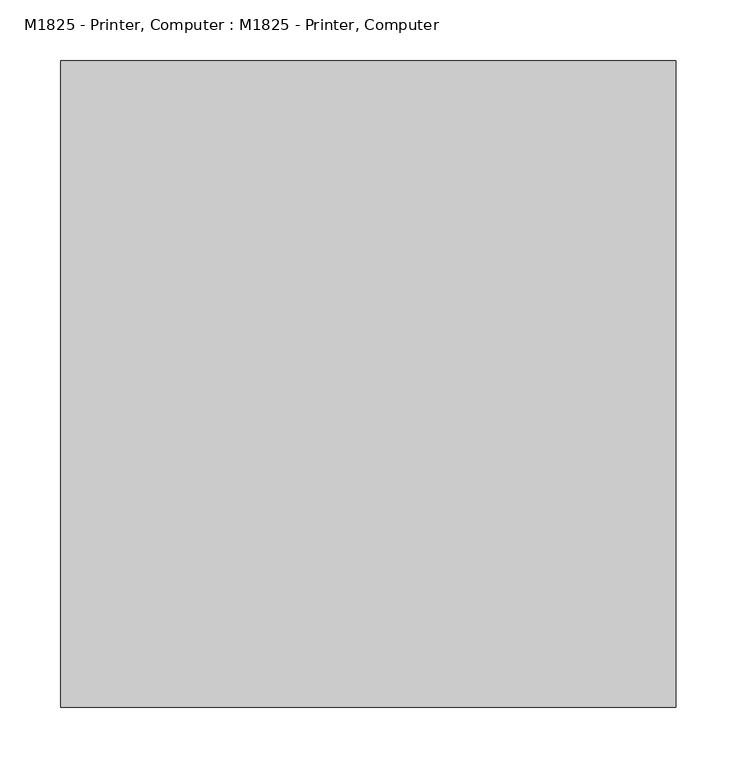
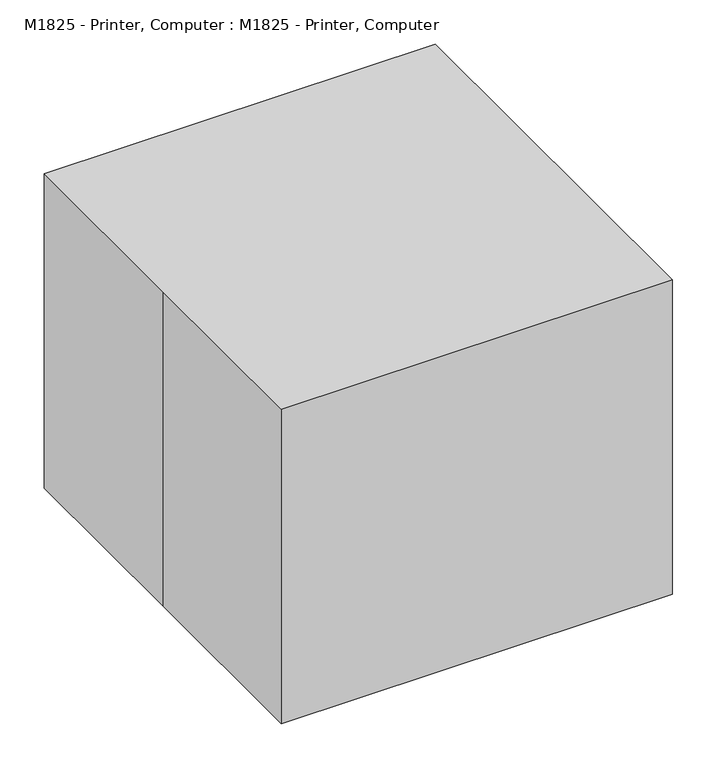
"""IFC4 building model written with IfcOpenShell, lengths in millimetres: proxy geometry, M1825 - Printer, Computer : M1825 - Printer, Computer."""

import ifcopenshell
import ifcopenshell.guid

model = None  # the IFC model being written
_history = None  # IfcOwnerHistory: only IFC2X3 demands one
_inside = {}  # id of a spatial element -> (the spatial element, [elements in it])
_under = {}  # id of a project, library or spatial element -> (it, [spatial elements below it])
_declared = {}  # id of a project -> (the project, [libraries it declares])
_typed = {}  # id of a type object -> (the type object, [elements of that type])
_made_of = {}  # id of a material, layer set ... -> (it, [elements and type objects made of it])


def new_model(schema):
    """Start an empty IFC model of exactly this schema.

    Asked for "IFC4X3", IfcOpenShell would pick the latest addendum, in which some entities
    have other attributes; the version numbers below select the first issue.
    IFC2X3 requires an IfcOwnerHistory on every rooted entity: one is made here for all.
    """
    global model, _history
    if schema == "IFC4X3":
        model = ifcopenshell.file(schema_version=(4, 3, 0, 0))
    else:
        model = ifcopenshell.file(schema=schema)
    _inside.clear()
    _under.clear()
    _declared.clear()
    _typed.clear()
    _made_of.clear()
    _history = None
    if model.schema == "IFC2X3":
        org = make("IfcOrganization", Name="unknown")
        user = make(
            "IfcPersonAndOrganization",
            ThePerson=make("IfcPerson", FamilyName="unknown"),
            TheOrganization=org,
        )
        app = make(
            "IfcApplication",
            ApplicationDeveloper=org,
            Version="unknown",
            ApplicationFullName="unknown",
            ApplicationIdentifier="unknown",
        )
        _history = make(
            "IfcOwnerHistory",
            OwningUser=user,
            OwningApplication=app,
            ChangeAction="ADDED",
            CreationDate=0,
        )
    return model


def make(cls, **values):
    """One entity of the class cls with the attributes given. An attribute that is None is left unset."""
    return model.create_entity(
        cls, **{name: value for name, value in values.items() if value is not None}
    )


def rooted(cls, **values):
    """An entity with a GlobalId (a new one), such as an element, a storey or a relation."""
    return make(cls, GlobalId=ifcopenshell.guid.new(), OwnerHistory=_history, **values)


def si_unit(unit_type, name, prefix=None):
    """IfcSIUnit, for example si_unit("LENGTHUNIT", "METRE", prefix="MILLI")."""
    return make("IfcSIUnit", UnitType=unit_type, Prefix=prefix, Name=name)


def assignment(units):
    """IfcUnitAssignment: the units of a project."""
    return None if units is None else make("IfcUnitAssignment", Units=units)


def point(xyz):
    """IfcCartesianPoint."""
    return None if xyz is None else make("IfcCartesianPoint", Coordinates=xyz)


def direction(xyz):
    """IfcDirection."""
    return None if xyz is None else make("IfcDirection", DirectionRatios=xyz)


def frame(location, z_axis=None, x_axis=None):
    """IfcAxis2Placement3D, a coordinate frame: its origin and axes. An axis left out is left unset."""
    return make(
        "IfcAxis2Placement3D",
        Location=point(location),
        Axis=direction(z_axis),
        RefDirection=direction(x_axis),
    )


def origin():
    """The frame at (0, 0, 0) with its axes left unset."""
    return frame((0.0, 0.0, 0.0))


def origin_with_axes():
    """The frame at (0, 0, 0) with the z axis (0, 0, 1) and the x axis (1, 0, 0) written out."""
    return frame((0.0, 0.0, 0.0), z_axis=(0.0, 0.0, 1.0), x_axis=(1.0, 0.0, 0.0))


def place(relative_to, where):
    """IfcLocalPlacement: puts the frame where relative to a parent placement (None: the world)."""
    return make(
        "IfcLocalPlacement", PlacementRelTo=relative_to, RelativePlacement=where
    )


def context(
    kind, dimensions, precision=None, world=None, true_north=None, identifier=None
):
    """IfcGeometricRepresentationContext, for example the 3D "Model" context."""
    return make(
        "IfcGeometricRepresentationContext",
        ContextIdentifier=identifier,
        ContextType=kind,
        CoordinateSpaceDimension=dimensions,
        Precision=precision,
        WorldCoordinateSystem=world,
        TrueNorth=true_north,
    )


def project(units=None, contexts=None):
    """IfcProject with its units and contexts."""
    return rooted(
        "IfcProject",
        Name="project",
        RepresentationContexts=contexts,
        UnitsInContext=assignment(units),
    )


def spatial(cls, under=None, at=None, **own):
    """A site, building, storey or space (cls), placed at a placement, below another one or the project."""
    s = rooted(cls, ObjectPlacement=at, **own)
    if under is not None:
        _under.setdefault(under.id(), (under, []))[1].append(s)
    return s


def polyline(points):
    """IfcPolyline through the points."""
    return make("IfcPolyline", Points=[point(p) for p in points])


def outline(outer, holes=None, kind="AREA"):
    """IfcArbitraryClosedProfileDef: a profile drawn as a closed curve; with holes, ...WithVoids."""
    if holes is None:
        return make("IfcArbitraryClosedProfileDef", ProfileType=kind, OuterCurve=outer)
    return make(
        "IfcArbitraryProfileDefWithVoids",
        ProfileType=kind,
        OuterCurve=outer,
        InnerCurves=holes,
    )


def extrude(swept, where, along, depth):
    """IfcExtrudedAreaSolid: the profile swept, set in the frame where, extruded along a direction by depth."""
    return make(
        "IfcExtrudedAreaSolid",
        SweptArea=swept,
        Position=where,
        ExtrudedDirection=direction(along),
        Depth=depth,
    )


def faces_of(points, faces, orient=None, outer=None):
    """IfcFace entities. A face is a list of loops; a loop is a list of indices into points, from 0.

    orient and outer hold one flag for each loop. By default every Orientation is true, the
    first loop of a face is its IfcFaceOuterBound and the others are IfcFaceBound.
    """
    made = []
    for i, loops in enumerate(faces):
        bounds = []
        for j, loop in enumerate(loops):
            is_outer = j == 0 if outer is None else outer[i][j]
            bounds.append(
                make(
                    "IfcFaceOuterBound" if is_outer else "IfcFaceBound",
                    Bound=make("IfcPolyLoop", Polygon=[points[k] for k in loop]),
                    Orientation=True if orient is None else orient[i][j],
                )
            )
        made.append(make("IfcFace", Bounds=bounds))
    return made


def faceted_brep(points, faces, orient=None, outer=None, voids=None):
    """IfcFacetedBrep: a solid bounded by flat faces; with voids (closed shells), ...WithVoids."""
    shared = [point(p) for p in points]
    hull = make("IfcClosedShell", CfsFaces=faces_of(shared, faces, orient, outer))
    if voids is None:
        return make("IfcFacetedBrep", Outer=hull)
    return make(
        "IfcFacetedBrepWithVoids",
        Outer=hull,
        Voids=[
            make(cls, CfsFaces=faces_of(shared, fs, o, b)) for cls, fs, o, b in voids
        ],
    )


def shape(context_of_items, identifier, shape_type, items):
    """IfcShapeRepresentation: the items that make up one representation, for example the "Body"."""
    return make(
        "IfcShapeRepresentation",
        ContextOfItems=context_of_items,
        RepresentationIdentifier=identifier,
        RepresentationType=shape_type,
        Items=items,
    )


def source(mapping_origin, context_of_items, identifier, shape_type, items):
    """IfcRepresentationMap: a shape defined once, which mapped items show again and again."""
    return make(
        "IfcRepresentationMap",
        MappingOrigin=mapping_origin,
        MappedRepresentation=shape(context_of_items, identifier, shape_type, items),
    )


def transform(
    local_origin,
    x_axis=None,
    y_axis=None,
    z_axis=None,
    scale=None,
    scale2=None,
    scale3=None,
    uniform=True,
):
    """IfcCartesianTransformationOperator3D, or its non-uniform kind. x_axis, y_axis, z_axis: its Axis1, 2, 3."""
    if uniform:
        return make(
            "IfcCartesianTransformationOperator3D",
            Axis1=direction(x_axis),
            Axis2=direction(y_axis),
            LocalOrigin=point(local_origin),
            Scale=scale,
            Axis3=direction(z_axis),
        )
    return make(
        "IfcCartesianTransformationOperator3DnonUniform",
        Axis1=direction(x_axis),
        Axis2=direction(y_axis),
        LocalOrigin=point(local_origin),
        Scale=scale,
        Axis3=direction(z_axis),
        Scale2=scale2,
        Scale3=scale3,
    )


def mapped(mapping_source, mapping_target):
    """IfcMappedItem: shows the shape of a source again, moved by a transform."""
    return make(
        "IfcMappedItem", MappingSource=mapping_source, MappingTarget=mapping_target
    )


def made_of(thing, what):
    """Note that an element or type object is made of a material, layer set ...; save() writes the relation."""
    if what is not None:
        _made_of.setdefault(what.id(), (what, []))[1].append(thing)
    return thing


def element(
    cls,
    number,
    at=None,
    inside=None,
    cuts=None,
    type_object=None,
    material=None,
    context=None,
    identifier="Body",
    shape_type=None,
    held_by="IfcProductDefinitionShape",
    body=None,
    shapes=None,
    **own,
):
    """One element of the class cls, such as IfcWall. Its Tag is "e" and its number.

    at: its placement. inside: the storey or other place that contains it. cuts: it is an
    opening in that element (IfcRelVoidsElement). A single representation is given by context,
    identifier, shape_type and body (its items); several are given by shapes. held_by: the class
    of the entity that holds the representations. save() writes the other relations.
    """
    e = rooted(cls, Tag="e%d" % number, ObjectPlacement=at, **own)
    if body is not None:
        shapes = [shape(context, identifier, shape_type, body)]
    if shapes is not None:
        e.Representation = make(held_by, Representations=shapes)
    if inside is not None:
        _inside.setdefault(inside.id(), (inside, []))[1].append(e)
    if cuts is not None:
        rooted(
            "IfcRelVoidsElement", RelatingBuildingElement=cuts, RelatedOpeningElement=e
        )
    if type_object is not None:
        _typed.setdefault(type_object.id(), (type_object, []))[1].append(e)
    return made_of(e, material)


def aggregate(whole, parts):
    """IfcRelAggregates: a whole, such as a stair, and the parts it consists of."""
    return rooted("IfcRelAggregates", RelatingObject=whole, RelatedObjects=parts)


def save(model, path):
    """Write the relations noted so far, then the file.

    IfcRelAggregates (storeys below a building ...), IfcRelContainedInSpatialStructure (elements
    in a storey), IfcRelDefinesByType, IfcRelAssociatesMaterial and IfcRelDeclares: one each for
    every whole, place, type object, material and project.
    """
    for whole, parts in _under.values():
        aggregate(whole, parts)
    for where, things in _inside.values():
        rooted(
            "IfcRelContainedInSpatialStructure",
            RelatedElements=things,
            RelatingStructure=where,
        )
    for kind, things in _typed.values():
        rooted("IfcRelDefinesByType", RelatedObjects=things, RelatingType=kind)
    for what, things in _made_of.values():
        rooted("IfcRelAssociatesMaterial", RelatedObjects=things, RelatingMaterial=what)
    for by, libraries in _declared.values():
        rooted("IfcRelDeclares", RelatingContext=by, RelatedDefinitions=libraries)
    model.write(path)


def m1825_printer_computer_m1825_printer_computer_fc716d7c(model_context):
    return source(origin(), model_context, "Body", "SolidModel", [
        faceted_brep([(215.9, 254.0, 355.6), (0.0, 254.0, 355.6), (0.0, -177.2046875, 355.6), (215.9, -177.2046875, 355.6), (-215.9, 254.0, 0.0), (215.9, 254.0, 0.0), (215.9, -177.2046875, 0.0), (-215.9, -177.2046875, 0.0), (-215.9, 254.0, 120.700198), (0.0, 254.0, 82.2650526), (0.0, 254.0, 177.8), (-215.9, 254.0, 177.8), (-215.9, 254.0, 322.8074523), (0.0, 254.0, 322.8074523), (-215.9, -177.2046875, 120.700198), (-215.9, 195.4931114, 322.8074523), (-215.9, -254.0, 177.8), (-215.9, -254.0, 254.0), (-215.9, -177.2046875, 254.0), (-215.9, -177.2046875, 322.8074523), (-215.9, -129.5796875, 322.8074523), (-215.9, -129.5796875, 254.0), (-215.9, 195.4931114, 254.0), (215.9, -254.0, 254.0), (215.9, -254.0, 177.8), (215.9, -177.2046875, 254.0), (215.9, -177.2046875, 177.8), (0.0, 195.4931114, 322.8074523), (0.0, -129.5796875, 322.8074523), (0.0, -177.2046875, 322.8074523), (0.0, 195.4931114, 254.0), (0.0, -129.5796875, 254.0), (0.0, -177.2046875, 177.8), (0.0, -177.2046875, 82.2650526)], [[[0, 1, 2, 3]], [[4, 5, 6, 7]], [[5, 4, 8, 9, 10, 11, 12, 13, 1, 0]], [[8, 4, 7, 14]], [[15, 12, 11, 16, 17, 18, 19, 20, 21, 22]], [[23, 17, 16, 24]], [[5, 0, 3, 25, 23, 24, 26, 6]], [[13, 12, 15, 27]], [[28, 20, 19, 29]], [[1, 13, 27, 30, 31, 28, 29, 2]], [[31, 21, 20, 28]], [[31, 30, 22, 21]], [[22, 30, 27, 15]], [[25, 18, 17, 23]], [[18, 25, 3, 2, 29, 19]], [[11, 10, 32, 26, 24, 16]], [[9, 8, 14, 33]], [[10, 9, 33, 32]], [[26, 32, 33, 14, 7, 6]]]),
        extrude(outline(polyline([(-254.0, 266.7), (254.0, 266.7), (254.0, -266.7), (-254.0, -266.7), (-254.0, 0.0), (-254.0, 266.7)])), origin_with_axes(), (0.0, 0.0, 1.0), 431.8),
    ])


if __name__ == "__main__":
    model = new_model("IFC4")
    model_context = context("Model", 3, world=origin())
    ifc_project = project(units=[si_unit("LENGTHUNIT", "METRE", prefix="MILLI")], contexts=[model_context])
    site = spatial("IfcSite", under=ifc_project)
    building = spatial("IfcBuilding", under=site)
    placement = place(None, origin())
    m1825_printer_computer_m1825_printer_computer_shape = m1825_printer_computer_m1825_printer_computer_fc716d7c(model_context)
    element("IfcBuildingElementProxy", 1, Name="M1825 - Printer, Computer : M1825 - Printer, Computer", ObjectType="M1825 - Printer, Computer : M1825 - Printer, Computer", at=placement, inside=building, context=model_context, shape_type="MappedRepresentation", body=[
        mapped(m1825_printer_computer_m1825_printer_computer_shape, transform((0.0, 0.0, 0.0), x_axis=(1.0, 0.0, 0.0), y_axis=(0.0, 1.0, 0.0), z_axis=(0.0, 0.0, 1.0))),
    ])
    save(model, "model.ifc")

# Revit data of these elements
# Type "M1825 - Printer, Computer : M1825 - Printer, Computer"
#   Watts2 = "0"
#   Watts1 = "690"
#   Unit_Issue = "EA"
#   UTIL_6_Misc = "-"
#   UTIL_5_NonMedGas = "-"
#   UTIL_4_MiscGas = "-"
#   UTIL_3_MedGas = "-"
#   UTIL_2_Elec = "A"
#   UTIL_1_WaterDrain = "-"
#   Nomenclature = "Printer, Computer"
#   NSN = "7025"
#   Location [instance default] = ""
#   JSN = "M1825"
#   Fund_Source_VA = "-"
#   Fund_Source_Navy = "-"
#   Fund_Source_Army = "-"
#   Fund_Source_AF = "-"
#   ELEC_Volts2 = "0"
#   ELEC_Volts1 = "120"
#   ELEC_Phase2 = "0"
#   ELEC_Phase1 = "1"
#   ELEC_HertzSwitch = "0"
#   ELEC_HertzDependent = "-1"
#   ELEC_Hertz = "60"
#   ELEC_Amps2 = "0"
#   ELEC_Amps1 = "3"
#   DetailDescription = "High resolution computer printer with a variety of type styles and sheet/envelope feeder trays. Database information reflects network ready, medium duty office style laser printers. Other types of printers (bubble jet, dot matrix, line or plotter) as well as light or heavy use capabilities are available."
#   CAT_VA = "C"
#   CAT_Navy = "C"
#   CAT_IHS = "-"
#   CAT_Army = "C"
#   CAT_AF = "C"
#   BTUperhour = "0"
#   Weight_IP = 54
#   DIM_Width_IP = 1' - 8"
#   DIM_Height_IP = 1' - 5"
#   DIM_Depth_IP = 1' - 9"
#   finish [instance default] = none
#   Assembly Code = ""
# Element 1 (IfcBuildingElementProxy, "M1825 - Printer, Computer : M1825 - Printer, Computer")
#   Materials on its faces: "EquipSpace"
# Materials
#   "EquipSpace": class "Unassigned", colour RGB 221 217 195, transparency 0.5
